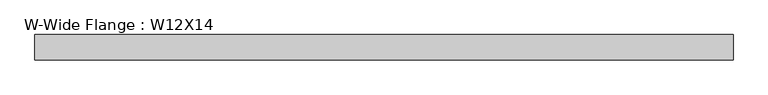
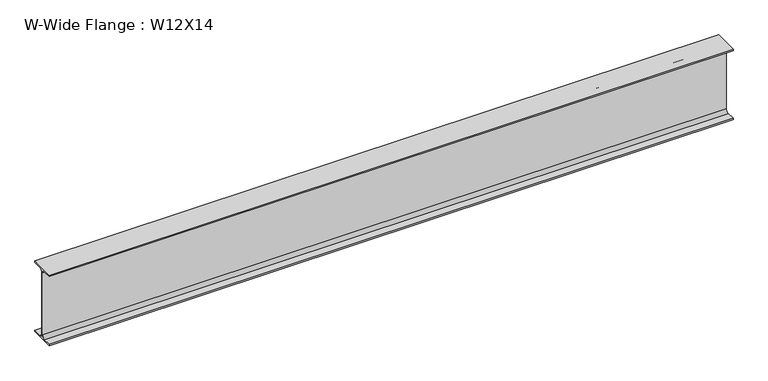
"""IFC4 building model written with IfcOpenShell, lengths in millimetres: beam geometry, W-Wide Flange : W12X14."""

from ifc_helpers import new_model, si_unit, point, frame, frame_2d, origin, place, context, project, spatial, polyline, circle_curve, trimmed, segment, composite_curve, outline, extrude, source, transform, mapped, element, save


def w_wide_flange_w12x14_3a621c7b(model_context):
    return source(origin(), model_context, "Body", "SweptSolid", [
        extrude(outline(composite_curve([segment(polyline([(50.419, -145.415), (50.419, -151.13), (-50.419, -151.13), (-50.419, -145.415), (-15.875, -145.415)]), True, "CONTINUOUS"), segment(trimmed(circle_curve(frame_2d((-15.875, -132.08)), 13.335), [point((-15.875, -145.415))], [point((-2.54, -132.08))], True, "CARTESIAN"), True, "CONTINUOUS"), segment(polyline([(-2.54, -132.08), (-2.54, 132.08)]), True, "CONTINUOUS"), segment(trimmed(circle_curve(frame_2d((-15.875, 132.08)), 13.335), [point((-2.54, 132.08))], [point((-15.875, 145.415))], True, "CARTESIAN"), True, "CONTINUOUS"), segment(polyline([(-15.875, 145.415), (-50.419, 145.415), (-50.419, 151.13), (50.419, 151.13), (50.419, 145.415), (15.875, 145.415)]), True, "CONTINUOUS"), segment(trimmed(circle_curve(frame_2d((15.875, 132.08)), 13.335), [point((15.875, 145.415))], [point((2.54, 132.08))], True, "CARTESIAN"), True, "CONTINUOUS"), segment(polyline([(2.54, 132.08), (2.54, -132.08)]), True, "CONTINUOUS"), segment(trimmed(circle_curve(frame_2d((15.875, -132.08)), 13.335), [point((2.54, -132.08))], [point((15.875, -145.415))], True, "CARTESIAN"), True, "CONTINUOUS"), segment(polyline([(15.875, -145.415), (50.419, -145.415)]), True, "CONTINUOUS")], self_intersect=False)), frame((-1384.2999994, 0.0, 0.0), z_axis=(1.0, 0.0, 0.0), x_axis=(0.0, 1.0, 0.0)), (0.0, 0.0, 1.0), 2768.5999988),
    ])


if __name__ == "__main__":
    model = new_model("IFC4")
    model_context = context("Model", 3, world=origin())
    ifc_project = project(units=[si_unit("LENGTHUNIT", "METRE", prefix="MILLI")], contexts=[model_context])
    site = spatial("IfcSite", under=ifc_project)
    building = spatial("IfcBuilding", under=site)
    placement = place(None, origin())
    w_wide_flange_w12x14_shape = w_wide_flange_w12x14_3a621c7b(model_context)
    element("IfcBeam", 1, ObjectType="W-Wide Flange : W12X14", at=placement, inside=building, context=model_context, shape_type="MappedRepresentation", body=[
        mapped(w_wide_flange_w12x14_shape, transform((0.0, 0.0, 0.0), x_axis=(1.0, 0.0, 0.0), y_axis=(0.0, 1.0, 0.0), z_axis=(0.0, 0.0, 1.0))),
    ])
    save(model, "model.ifc")

# Revit data of these elements
# Type "W-Wide Flange : W12X14"
#   Assembly Code = "B10"
#   W = 14
#   Length [instance default] = 5' - 0"
#   bf = 0' - 3.97"
#   d = 0' - 11.9"
#   k = 0' - 0 3/4"
#   k2 = 0' - 0.525"
#   tf = 0' - 0.225"
#   tw = 0' - 0.2"
#   A = 0.0288889 SF
#   Structural Material [instance default] = Steel ASTM A992
# Element 1 (IfcBeam, "W-Wide Flange : W12X14")
#   Materials on its faces: "Steel ASTM A992"
# Materials
#   "Steel ASTM A992": class "Metal", colour RGB 199 199 199, transparency 0, Description = "Structural steel 50ksi", Cost = 0
